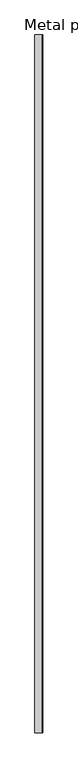
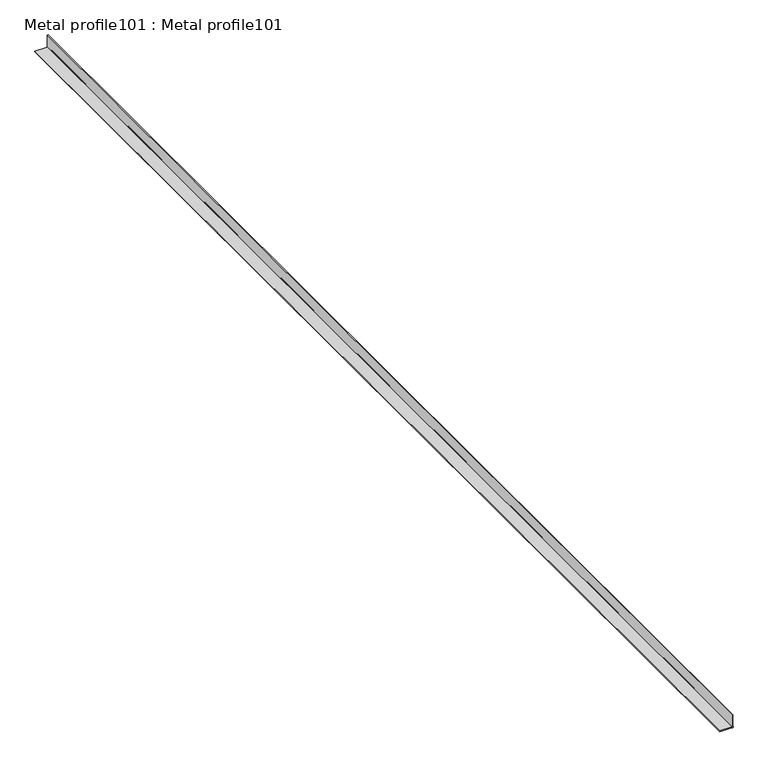
"""IFC4 building model written with IfcOpenShell, lengths in millimetres: proxy geometry, Metal profile101 : Metal profile101."""

import ifcopenshell
import ifcopenshell.guid

model = None  # the IFC model being written
_history = None  # IfcOwnerHistory: only IFC2X3 demands one
_inside = {}  # id of a spatial element -> (the spatial element, [elements in it])
_under = {}  # id of a project, library or spatial element -> (it, [spatial elements below it])
_declared = {}  # id of a project -> (the project, [libraries it declares])
_typed = {}  # id of a type object -> (the type object, [elements of that type])
_made_of = {}  # id of a material, layer set ... -> (it, [elements and type objects made of it])


def new_model(schema):
    """Start an empty IFC model of exactly this schema.

    Asked for "IFC4X3", IfcOpenShell would pick the latest addendum, in which some entities
    have other attributes; the version numbers below select the first issue.
    IFC2X3 requires an IfcOwnerHistory on every rooted entity: one is made here for all.
    """
    global model, _history
    if schema == "IFC4X3":
        model = ifcopenshell.file(schema_version=(4, 3, 0, 0))
    else:
        model = ifcopenshell.file(schema=schema)
    _inside.clear()
    _under.clear()
    _declared.clear()
    _typed.clear()
    _made_of.clear()
    _history = None
    if model.schema == "IFC2X3":
        org = make("IfcOrganization", Name="unknown")
        user = make(
            "IfcPersonAndOrganization",
            ThePerson=make("IfcPerson", FamilyName="unknown"),
            TheOrganization=org,
        )
        app = make(
            "IfcApplication",
            ApplicationDeveloper=org,
            Version="unknown",
            ApplicationFullName="unknown",
            ApplicationIdentifier="unknown",
        )
        _history = make(
            "IfcOwnerHistory",
            OwningUser=user,
            OwningApplication=app,
            ChangeAction="ADDED",
            CreationDate=0,
        )
    return model


def make(cls, **values):
    """One entity of the class cls with the attributes given. An attribute that is None is left unset."""
    return model.create_entity(
        cls, **{name: value for name, value in values.items() if value is not None}
    )


def rooted(cls, **values):
    """An entity with a GlobalId (a new one), such as an element, a storey or a relation."""
    return make(cls, GlobalId=ifcopenshell.guid.new(), OwnerHistory=_history, **values)


def si_unit(unit_type, name, prefix=None):
    """IfcSIUnit, for example si_unit("LENGTHUNIT", "METRE", prefix="MILLI")."""
    return make("IfcSIUnit", UnitType=unit_type, Prefix=prefix, Name=name)


def assignment(units):
    """IfcUnitAssignment: the units of a project."""
    return None if units is None else make("IfcUnitAssignment", Units=units)


def point(xyz):
    """IfcCartesianPoint."""
    return None if xyz is None else make("IfcCartesianPoint", Coordinates=xyz)


def direction(xyz):
    """IfcDirection."""
    return None if xyz is None else make("IfcDirection", DirectionRatios=xyz)


def frame(location, z_axis=None, x_axis=None):
    """IfcAxis2Placement3D, a coordinate frame: its origin and axes. An axis left out is left unset."""
    return make(
        "IfcAxis2Placement3D",
        Location=point(location),
        Axis=direction(z_axis),
        RefDirection=direction(x_axis),
    )


def frame_2d(location, x_axis=None):
    """IfcAxis2Placement2D, a coordinate frame in the plane: its origin and x axis."""
    return make(
        "IfcAxis2Placement2D", Location=point(location), RefDirection=direction(x_axis)
    )


def origin():
    """The frame at (0, 0, 0) with its axes left unset."""
    return frame((0.0, 0.0, 0.0))


def place(relative_to, where):
    """IfcLocalPlacement: puts the frame where relative to a parent placement (None: the world)."""
    return make(
        "IfcLocalPlacement", PlacementRelTo=relative_to, RelativePlacement=where
    )


def context(
    kind, dimensions, precision=None, world=None, true_north=None, identifier=None
):
    """IfcGeometricRepresentationContext, for example the 3D "Model" context."""
    return make(
        "IfcGeometricRepresentationContext",
        ContextIdentifier=identifier,
        ContextType=kind,
        CoordinateSpaceDimension=dimensions,
        Precision=precision,
        WorldCoordinateSystem=world,
        TrueNorth=true_north,
    )


def project(units=None, contexts=None):
    """IfcProject with its units and contexts."""
    return rooted(
        "IfcProject",
        Name="project",
        RepresentationContexts=contexts,
        UnitsInContext=assignment(units),
    )


def spatial(cls, under=None, at=None, **own):
    """A site, building, storey or space (cls), placed at a placement, below another one or the project."""
    s = rooted(cls, ObjectPlacement=at, **own)
    if under is not None:
        _under.setdefault(under.id(), (under, []))[1].append(s)
    return s


def polyline(points):
    """IfcPolyline through the points."""
    return make("IfcPolyline", Points=[point(p) for p in points])


def circle_curve(where, radius):
    """IfcCircle in the frame where."""
    return make("IfcCircle", Position=where, Radius=radius)


def trimmed(basis, trim1, trim2, sense, master):
    """IfcTrimmedCurve: the piece of a basis curve between two trims."""
    return make(
        "IfcTrimmedCurve",
        BasisCurve=basis,
        Trim1=trim1,
        Trim2=trim2,
        SenseAgreement=sense,
        MasterRepresentation=master,
    )


def segment(curve, same_sense, transition):
    """IfcCompositeCurveSegment."""
    return make(
        "IfcCompositeCurveSegment",
        Transition=transition,
        SameSense=same_sense,
        ParentCurve=curve,
    )


def composite_curve(segments, self_intersect=None):
    """IfcCompositeCurve: segments joined end to end."""
    return make("IfcCompositeCurve", Segments=segments, SelfIntersect=self_intersect)


def outline(outer, holes=None, kind="AREA"):
    """IfcArbitraryClosedProfileDef: a profile drawn as a closed curve; with holes, ...WithVoids."""
    if holes is None:
        return make("IfcArbitraryClosedProfileDef", ProfileType=kind, OuterCurve=outer)
    return make(
        "IfcArbitraryProfileDefWithVoids",
        ProfileType=kind,
        OuterCurve=outer,
        InnerCurves=holes,
    )


def extrude(swept, where, along, depth):
    """IfcExtrudedAreaSolid: the profile swept, set in the frame where, extruded along a direction by depth."""
    return make(
        "IfcExtrudedAreaSolid",
        SweptArea=swept,
        Position=where,
        ExtrudedDirection=direction(along),
        Depth=depth,
    )


def shape(context_of_items, identifier, shape_type, items):
    """IfcShapeRepresentation: the items that make up one representation, for example the "Body"."""
    return make(
        "IfcShapeRepresentation",
        ContextOfItems=context_of_items,
        RepresentationIdentifier=identifier,
        RepresentationType=shape_type,
        Items=items,
    )


def source(mapping_origin, context_of_items, identifier, shape_type, items):
    """IfcRepresentationMap: a shape defined once, which mapped items show again and again."""
    return make(
        "IfcRepresentationMap",
        MappingOrigin=mapping_origin,
        MappedRepresentation=shape(context_of_items, identifier, shape_type, items),
    )


def transform(
    local_origin,
    x_axis=None,
    y_axis=None,
    z_axis=None,
    scale=None,
    scale2=None,
    scale3=None,
    uniform=True,
):
    """IfcCartesianTransformationOperator3D, or its non-uniform kind. x_axis, y_axis, z_axis: its Axis1, 2, 3."""
    if uniform:
        return make(
            "IfcCartesianTransformationOperator3D",
            Axis1=direction(x_axis),
            Axis2=direction(y_axis),
            LocalOrigin=point(local_origin),
            Scale=scale,
            Axis3=direction(z_axis),
        )
    return make(
        "IfcCartesianTransformationOperator3DnonUniform",
        Axis1=direction(x_axis),
        Axis2=direction(y_axis),
        LocalOrigin=point(local_origin),
        Scale=scale,
        Axis3=direction(z_axis),
        Scale2=scale2,
        Scale3=scale3,
    )


def mapped(mapping_source, mapping_target):
    """IfcMappedItem: shows the shape of a source again, moved by a transform."""
    return make(
        "IfcMappedItem", MappingSource=mapping_source, MappingTarget=mapping_target
    )


def made_of(thing, what):
    """Note that an element or type object is made of a material, layer set ...; save() writes the relation."""
    if what is not None:
        _made_of.setdefault(what.id(), (what, []))[1].append(thing)
    return thing


def element(
    cls,
    number,
    at=None,
    inside=None,
    cuts=None,
    type_object=None,
    material=None,
    context=None,
    identifier="Body",
    shape_type=None,
    held_by="IfcProductDefinitionShape",
    body=None,
    shapes=None,
    **own,
):
    """One element of the class cls, such as IfcWall. Its Tag is "e" and its number.

    at: its placement. inside: the storey or other place that contains it. cuts: it is an
    opening in that element (IfcRelVoidsElement). A single representation is given by context,
    identifier, shape_type and body (its items); several are given by shapes. held_by: the class
    of the entity that holds the representations. save() writes the other relations.
    """
    e = rooted(cls, Tag="e%d" % number, ObjectPlacement=at, **own)
    if body is not None:
        shapes = [shape(context, identifier, shape_type, body)]
    if shapes is not None:
        e.Representation = make(held_by, Representations=shapes)
    if inside is not None:
        _inside.setdefault(inside.id(), (inside, []))[1].append(e)
    if cuts is not None:
        rooted(
            "IfcRelVoidsElement", RelatingBuildingElement=cuts, RelatedOpeningElement=e
        )
    if type_object is not None:
        _typed.setdefault(type_object.id(), (type_object, []))[1].append(e)
    return made_of(e, material)


def aggregate(whole, parts):
    """IfcRelAggregates: a whole, such as a stair, and the parts it consists of."""
    return rooted("IfcRelAggregates", RelatingObject=whole, RelatedObjects=parts)


def save(model, path):
    """Write the relations noted so far, then the file.

    IfcRelAggregates (storeys below a building ...), IfcRelContainedInSpatialStructure (elements
    in a storey), IfcRelDefinesByType, IfcRelAssociatesMaterial and IfcRelDeclares: one each for
    every whole, place, type object, material and project.
    """
    for whole, parts in _under.values():
        aggregate(whole, parts)
    for where, things in _inside.values():
        rooted(
            "IfcRelContainedInSpatialStructure",
            RelatedElements=things,
            RelatingStructure=where,
        )
    for kind, things in _typed.values():
        rooted("IfcRelDefinesByType", RelatedObjects=things, RelatingType=kind)
    for what, things in _made_of.values():
        rooted("IfcRelAssociatesMaterial", RelatedObjects=things, RelatingMaterial=what)
    for by, libraries in _declared.values():
        rooted("IfcRelDeclares", RelatingContext=by, RelatedDefinitions=libraries)
    model.write(path)


def metal_profile101_metal_profile101_1afb723c(model_context):
    return source(origin(), model_context, "Body", "SweptSolid", [
        extrude(outline(composite_curve([segment(polyline([(35055.7175625, -8274.3138807), (35054.4375625, -8274.3138807), (35054.4375625, -8253.410971)]), True, "CONTINUOUS"), segment(trimmed(circle_curve(frame_2d((35055.0775625, -8252.5206967)), 1.0964434), [point((35054.4375625, -8253.410971))], [point((35055.9678367, -8251.8806967))], False, "CARTESIAN"), True, "CONTINUOUS"), segment(polyline([(35055.9678367, -8251.8806967), (35076.8707464, -8251.8806967), (35076.8707464, -8253.1606967), (35055.7175625, -8253.1606967), (35055.7175625, -8274.3138807)]), True, "CONTINUOUS")], self_intersect=False)), frame((0.0, 4540.4513244, 0.0), z_axis=(0.0, 1.0, 0.0), x_axis=(0.0, 0.0, 1.0)), (0.0, 0.0, 1.0), 2000.0),
    ])


if __name__ == "__main__":
    model = new_model("IFC4")
    model_context = context("Model", 3, world=origin())
    ifc_project = project(units=[si_unit("LENGTHUNIT", "METRE", prefix="MILLI")], contexts=[model_context])
    site = spatial("IfcSite", under=ifc_project)
    building = spatial("IfcBuilding", under=site)
    placement = place(None, origin())
    metal_profile101_metal_profile101_shape = metal_profile101_metal_profile101_1afb723c(model_context)
    element("IfcBuildingElementProxy", 1, Name="Metal profile101 : Metal profile101", ObjectType="Metal profile101 : Metal profile101", at=placement, inside=building, context=model_context, shape_type="MappedRepresentation", body=[
        mapped(metal_profile101_metal_profile101_shape, transform((0.0, 0.0, 0.0), x_axis=(1.0, 0.0, 0.0), y_axis=(0.0, 1.0, 0.0), z_axis=(0.0, 0.0, 1.0))),
    ])
    save(model, "model.ifc")

# Revit data of these elements
# Type "Metal profile101 : Metal profile101"
#   NameOverride = "Metal profile101"
# Element 1 (IfcBuildingElementProxy, "Metal profile101 : Metal profile101")
#   Materials on its faces: "CORNER BEAD"
# Materials
#   "CORNER BEAD": class "Unassigned", colour RGB 253 236 176, transparency 0, Cost = 0
